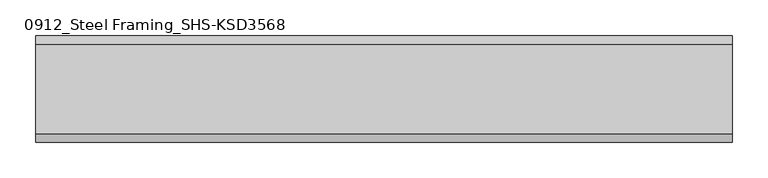
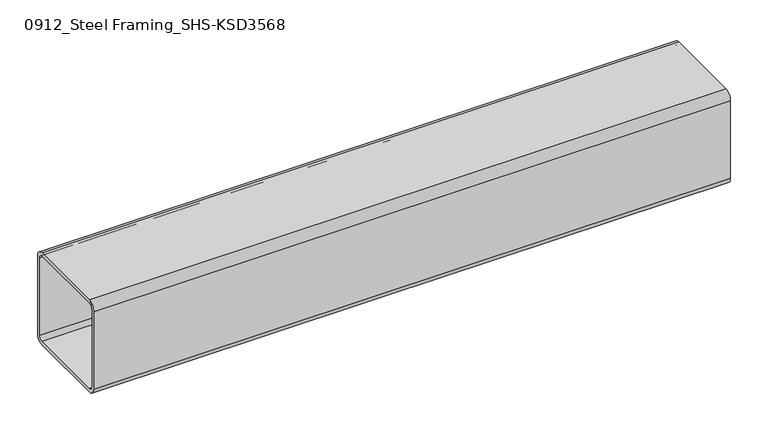
"""IFC4 building model written with IfcOpenShell, lengths in millimetres: beam geometry, 0912_Steel Framing_SHS-KSD3568 : H_SB_ASB_SHS-150x150x6."""

from ifc_helpers import new_model, si_unit, point, frame, frame_2d, origin, place, context, project, spatial, polyline, circle_curve, trimmed, segment, composite_curve, outline, extrude, source, transform, mapped, element, save


def beam_0912_steel_framing_shs_ksd3568_c83f5935(model_context):
    return source(origin(), model_context, "Body", "SweptSolid", [
        extrude(outline(composite_curve([segment(polyline([(75.0, 63.0), (75.0, -63.0)]), True, "CONTINUOUS"), segment(trimmed(circle_curve(frame_2d((63.0, -63.0)), 12.0), [point((75.0, -63.0))], [point((63.0, -75.0))], False, "CARTESIAN"), True, "CONTINUOUS"), segment(polyline([(63.0, -75.0), (-63.0, -75.0)]), True, "CONTINUOUS"), segment(trimmed(circle_curve(frame_2d((-63.0, -63.0)), 12.0), [point((-63.0, -75.0))], [point((-75.0, -63.0))], False, "CARTESIAN"), True, "CONTINUOUS"), segment(polyline([(-75.0, -63.0), (-75.0, 63.0)]), True, "CONTINUOUS"), segment(trimmed(circle_curve(frame_2d((-63.0, 63.0)), 12.0), [point((-75.0, 63.0))], [point((-63.0, 75.0))], False, "CARTESIAN"), True, "CONTINUOUS"), segment(polyline([(-63.0, 75.0), (63.0, 75.0)]), True, "CONTINUOUS"), segment(trimmed(circle_curve(frame_2d((63.0, 63.0)), 12.0), [point((63.0, 75.0))], [point((75.0, 63.0))], False, "CARTESIAN"), True, "CONTINUOUS")], self_intersect=False), holes=[composite_curve([segment(trimmed(circle_curve(frame_2d((-63.0, 63.0)), 6.0), [point((-63.0, 69.0))], [point((-69.0, 63.0))], True, "CARTESIAN"), True, "CONTINUOUS"), segment(polyline([(-69.0, 63.0), (-69.0, -63.0)]), True, "CONTINUOUS"), segment(trimmed(circle_curve(frame_2d((-63.0, -63.0)), 6.0), [point((-69.0, -63.0))], [point((-63.0, -69.0))], True, "CARTESIAN"), True, "CONTINUOUS"), segment(polyline([(-63.0, -69.0), (63.0, -69.0)]), True, "CONTINUOUS"), segment(trimmed(circle_curve(frame_2d((63.0, -63.0)), 6.0), [point((63.0, -69.0))], [point((69.0, -63.0))], True, "CARTESIAN"), True, "CONTINUOUS"), segment(polyline([(69.0, -63.0), (69.0, 63.0)]), True, "CONTINUOUS"), segment(trimmed(circle_curve(frame_2d((63.0, 63.0)), 6.0), [point((69.0, 63.0))], [point((63.0, 69.0))], True, "CARTESIAN"), True, "CONTINUOUS"), segment(polyline([(63.0, 69.0), (-63.0, 69.0)]), True, "CONTINUOUS")], self_intersect=False)]), frame((-490.0, 0.0, 0.0), z_axis=(1.0, 0.0, 0.0), x_axis=(0.0, 1.0, 0.0)), (0.0, 0.0, 1.0), 980.0),
    ])


if __name__ == "__main__":
    model = new_model("IFC4")
    model_context = context("Model", 3, world=origin())
    ifc_project = project(units=[si_unit("LENGTHUNIT", "METRE", prefix="MILLI")], contexts=[model_context])
    site = spatial("IfcSite", under=ifc_project)
    building = spatial("IfcBuilding", under=site)
    placement = place(None, origin())
    beam_0912_steel_framing_shs_ksd3568_shape = beam_0912_steel_framing_shs_ksd3568_c83f5935(model_context)
    element("IfcBeam", 1, ObjectType="0912_Steel Framing_SHS-KSD3568 : H_SB_ASB_SHS-150x150x6", at=placement, inside=building, context=model_context, shape_type="MappedRepresentation", body=[
        mapped(beam_0912_steel_framing_shs_ksd3568_shape, transform((0.0, 0.0, 0.0), x_axis=(1.0, 0.0, 0.0), y_axis=(0.0, 1.0, 0.0), z_axis=(0.0, 0.0, 1.0))),
    ])
    save(model, "model.ifc")

# Revit data of these elements
# Type "0912_Steel Framing_SHS-KSD3568 : H_SB_ASB_SHS-150x150x6"
#   H_WM Code_1 = "S01AA002-00001 | Main Steel Structure Fabrication Work | Shelter/Building | Medium Steel - Standard (90KG/M>Weight≥30KG/M) | Material: (   )"
#   H_WM Code_2 = "S03AA028-00001 | Main Steel Structure Erection Work | Shelter/Building | Medium Steel (90KG/M>Weight≥30KG/M) | Material: (   )"
#   H_WM Code_3 = "S01AA010-00001 | Main Steel Structure Fabrication Work | Shelter/Building | Steel Painting/Coating | for Non-Fireproofed Steel Surface, Surface Preparation, Primer, Second & Final Coat | Material: (   )"
#   H_Q'ty Cal Type Tag = "SB-Q2"
#   Perimeter = 0.60 m²/m
#   Nominal Weight = 26.40 kgf/m
#   Length [instance default] = 1.0000 m
#   b = 0.1500 m
#   h = 0.1500 m
#   tr = 0.0120 m
#   t = 0.0060 m
#   A = 28.36 m²
#   Structural Material [instance default] = Steel, 45-345
# Element 1 (IfcBeam, "0912_Steel Framing_SHS-KSD3568 : H_SB_ASB_SHS-150x150x6")
#   Structural Material = none
# Materials
#   "Steel, 45-345": class "Metal", colour RGB 189 187 185, transparency 0, Description = "Steel 345 MPa", Cost = 0
